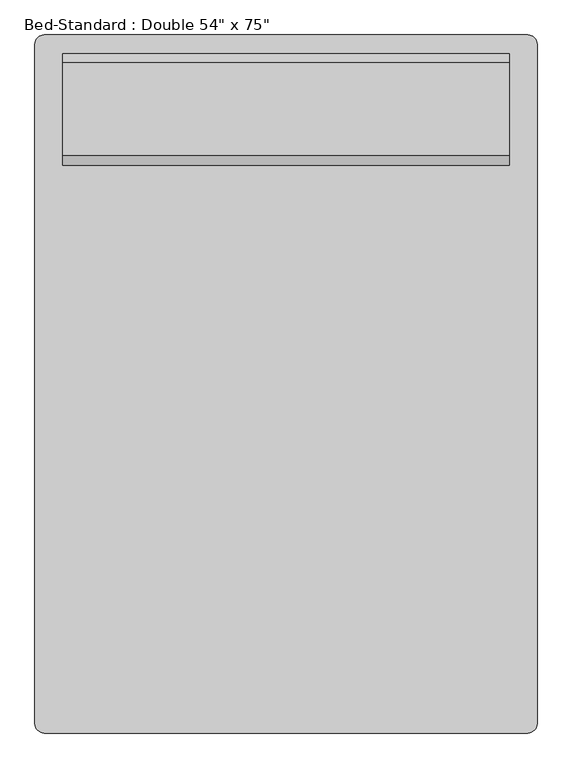
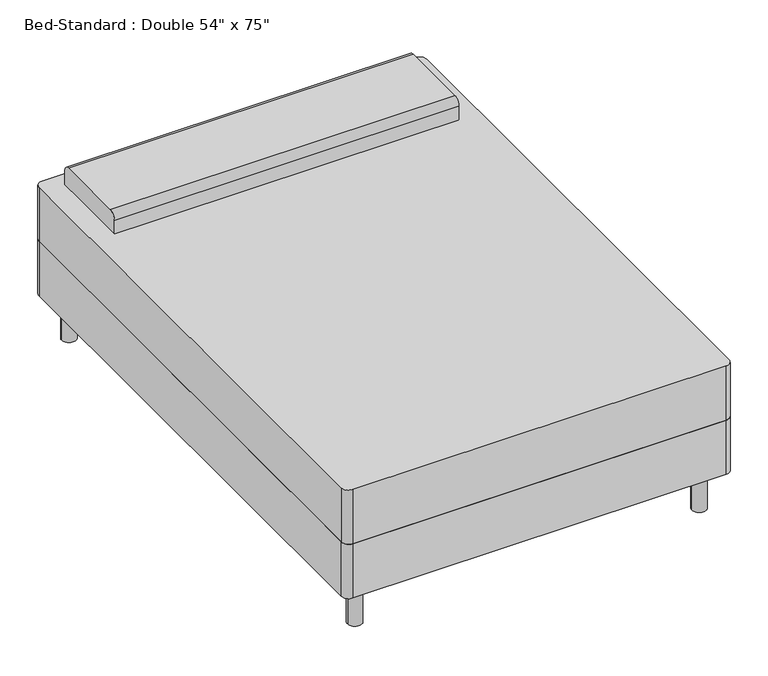
"""IFC4 building model written with IfcOpenShell, lengths in millimetres: furniture geometry."""

import ifcopenshell
import ifcopenshell.guid

model = None  # the IFC model being written
_history = None  # IfcOwnerHistory: only IFC2X3 demands one
_inside = {}  # id of a spatial element -> (the spatial element, [elements in it])
_under = {}  # id of a project, library or spatial element -> (it, [spatial elements below it])
_declared = {}  # id of a project -> (the project, [libraries it declares])
_typed = {}  # id of a type object -> (the type object, [elements of that type])
_made_of = {}  # id of a material, layer set ... -> (it, [elements and type objects made of it])


def new_model(schema):
    """Start an empty IFC model of exactly this schema.

    Asked for "IFC4X3", IfcOpenShell would pick the latest addendum, in which some entities
    have other attributes; the version numbers below select the first issue.
    IFC2X3 requires an IfcOwnerHistory on every rooted entity: one is made here for all.
    """
    global model, _history
    if schema == "IFC4X3":
        model = ifcopenshell.file(schema_version=(4, 3, 0, 0))
    else:
        model = ifcopenshell.file(schema=schema)
    _inside.clear()
    _under.clear()
    _declared.clear()
    _typed.clear()
    _made_of.clear()
    _history = None
    if model.schema == "IFC2X3":
        org = make("IfcOrganization", Name="unknown")
        user = make(
            "IfcPersonAndOrganization",
            ThePerson=make("IfcPerson", FamilyName="unknown"),
            TheOrganization=org,
        )
        app = make(
            "IfcApplication",
            ApplicationDeveloper=org,
            Version="unknown",
            ApplicationFullName="unknown",
            ApplicationIdentifier="unknown",
        )
        _history = make(
            "IfcOwnerHistory",
            OwningUser=user,
            OwningApplication=app,
            ChangeAction="ADDED",
            CreationDate=0,
        )
    return model


def make(cls, **values):
    """One entity of the class cls with the attributes given. An attribute that is None is left unset."""
    return model.create_entity(
        cls, **{name: value for name, value in values.items() if value is not None}
    )


def rooted(cls, **values):
    """An entity with a GlobalId (a new one), such as an element, a storey or a relation."""
    return make(cls, GlobalId=ifcopenshell.guid.new(), OwnerHistory=_history, **values)


def si_unit(unit_type, name, prefix=None):
    """IfcSIUnit, for example si_unit("LENGTHUNIT", "METRE", prefix="MILLI")."""
    return make("IfcSIUnit", UnitType=unit_type, Prefix=prefix, Name=name)


def assignment(units):
    """IfcUnitAssignment: the units of a project."""
    return None if units is None else make("IfcUnitAssignment", Units=units)


def point(xyz):
    """IfcCartesianPoint."""
    return None if xyz is None else make("IfcCartesianPoint", Coordinates=xyz)


def direction(xyz):
    """IfcDirection."""
    return None if xyz is None else make("IfcDirection", DirectionRatios=xyz)


def frame(location, z_axis=None, x_axis=None):
    """IfcAxis2Placement3D, a coordinate frame: its origin and axes. An axis left out is left unset."""
    return make(
        "IfcAxis2Placement3D",
        Location=point(location),
        Axis=direction(z_axis),
        RefDirection=direction(x_axis),
    )


def frame_2d(location, x_axis=None):
    """IfcAxis2Placement2D, a coordinate frame in the plane: its origin and x axis."""
    return make(
        "IfcAxis2Placement2D", Location=point(location), RefDirection=direction(x_axis)
    )


def origin():
    """The frame at (0, 0, 0) with its axes left unset."""
    return frame((0.0, 0.0, 0.0))


def origin_with_axes():
    """The frame at (0, 0, 0) with the z axis (0, 0, 1) and the x axis (1, 0, 0) written out."""
    return frame((0.0, 0.0, 0.0), z_axis=(0.0, 0.0, 1.0), x_axis=(1.0, 0.0, 0.0))


def place(relative_to, where):
    """IfcLocalPlacement: puts the frame where relative to a parent placement (None: the world)."""
    return make(
        "IfcLocalPlacement", PlacementRelTo=relative_to, RelativePlacement=where
    )


def context(
    kind, dimensions, precision=None, world=None, true_north=None, identifier=None
):
    """IfcGeometricRepresentationContext, for example the 3D "Model" context."""
    return make(
        "IfcGeometricRepresentationContext",
        ContextIdentifier=identifier,
        ContextType=kind,
        CoordinateSpaceDimension=dimensions,
        Precision=precision,
        WorldCoordinateSystem=world,
        TrueNorth=true_north,
    )


def project(units=None, contexts=None):
    """IfcProject with its units and contexts."""
    return rooted(
        "IfcProject",
        Name="project",
        RepresentationContexts=contexts,
        UnitsInContext=assignment(units),
    )


def spatial(cls, under=None, at=None, **own):
    """A site, building, storey or space (cls), placed at a placement, below another one or the project."""
    s = rooted(cls, ObjectPlacement=at, **own)
    if under is not None:
        _under.setdefault(under.id(), (under, []))[1].append(s)
    return s


def polyline(points):
    """IfcPolyline through the points."""
    return make("IfcPolyline", Points=[point(p) for p in points])


def circle_curve(where, radius):
    """IfcCircle in the frame where."""
    return make("IfcCircle", Position=where, Radius=radius)


def trimmed(basis, trim1, trim2, sense, master):
    """IfcTrimmedCurve: the piece of a basis curve between two trims."""
    return make(
        "IfcTrimmedCurve",
        BasisCurve=basis,
        Trim1=trim1,
        Trim2=trim2,
        SenseAgreement=sense,
        MasterRepresentation=master,
    )


def segment(curve, same_sense, transition):
    """IfcCompositeCurveSegment."""
    return make(
        "IfcCompositeCurveSegment",
        Transition=transition,
        SameSense=same_sense,
        ParentCurve=curve,
    )


def composite_curve(segments, self_intersect=None):
    """IfcCompositeCurve: segments joined end to end."""
    return make("IfcCompositeCurve", Segments=segments, SelfIntersect=self_intersect)


def outline(outer, holes=None, kind="AREA"):
    """IfcArbitraryClosedProfileDef: a profile drawn as a closed curve; with holes, ...WithVoids."""
    if holes is None:
        return make("IfcArbitraryClosedProfileDef", ProfileType=kind, OuterCurve=outer)
    return make(
        "IfcArbitraryProfileDefWithVoids",
        ProfileType=kind,
        OuterCurve=outer,
        InnerCurves=holes,
    )


def extrude(swept, where, along, depth):
    """IfcExtrudedAreaSolid: the profile swept, set in the frame where, extruded along a direction by depth."""
    return make(
        "IfcExtrudedAreaSolid",
        SweptArea=swept,
        Position=where,
        ExtrudedDirection=direction(along),
        Depth=depth,
    )


def shape(context_of_items, identifier, shape_type, items):
    """IfcShapeRepresentation: the items that make up one representation, for example the "Body"."""
    return make(
        "IfcShapeRepresentation",
        ContextOfItems=context_of_items,
        RepresentationIdentifier=identifier,
        RepresentationType=shape_type,
        Items=items,
    )


def source(mapping_origin, context_of_items, identifier, shape_type, items):
    """IfcRepresentationMap: a shape defined once, which mapped items show again and again."""
    return make(
        "IfcRepresentationMap",
        MappingOrigin=mapping_origin,
        MappedRepresentation=shape(context_of_items, identifier, shape_type, items),
    )


def transform(
    local_origin,
    x_axis=None,
    y_axis=None,
    z_axis=None,
    scale=None,
    scale2=None,
    scale3=None,
    uniform=True,
):
    """IfcCartesianTransformationOperator3D, or its non-uniform kind. x_axis, y_axis, z_axis: its Axis1, 2, 3."""
    if uniform:
        return make(
            "IfcCartesianTransformationOperator3D",
            Axis1=direction(x_axis),
            Axis2=direction(y_axis),
            LocalOrigin=point(local_origin),
            Scale=scale,
            Axis3=direction(z_axis),
        )
    return make(
        "IfcCartesianTransformationOperator3DnonUniform",
        Axis1=direction(x_axis),
        Axis2=direction(y_axis),
        LocalOrigin=point(local_origin),
        Scale=scale,
        Axis3=direction(z_axis),
        Scale2=scale2,
        Scale3=scale3,
    )


def mapped(mapping_source, mapping_target):
    """IfcMappedItem: shows the shape of a source again, moved by a transform."""
    return make(
        "IfcMappedItem", MappingSource=mapping_source, MappingTarget=mapping_target
    )


def made_of(thing, what):
    """Note that an element or type object is made of a material, layer set ...; save() writes the relation."""
    if what is not None:
        _made_of.setdefault(what.id(), (what, []))[1].append(thing)
    return thing


def element(
    cls,
    number,
    at=None,
    inside=None,
    cuts=None,
    type_object=None,
    material=None,
    context=None,
    identifier="Body",
    shape_type=None,
    held_by="IfcProductDefinitionShape",
    body=None,
    shapes=None,
    **own,
):
    """One element of the class cls, such as IfcWall. Its Tag is "e" and its number.

    at: its placement. inside: the storey or other place that contains it. cuts: it is an
    opening in that element (IfcRelVoidsElement). A single representation is given by context,
    identifier, shape_type and body (its items); several are given by shapes. held_by: the class
    of the entity that holds the representations. save() writes the other relations.
    """
    e = rooted(cls, Tag="e%d" % number, ObjectPlacement=at, **own)
    if body is not None:
        shapes = [shape(context, identifier, shape_type, body)]
    if shapes is not None:
        e.Representation = make(held_by, Representations=shapes)
    if inside is not None:
        _inside.setdefault(inside.id(), (inside, []))[1].append(e)
    if cuts is not None:
        rooted(
            "IfcRelVoidsElement", RelatingBuildingElement=cuts, RelatedOpeningElement=e
        )
    if type_object is not None:
        _typed.setdefault(type_object.id(), (type_object, []))[1].append(e)
    return made_of(e, material)


def aggregate(whole, parts):
    """IfcRelAggregates: a whole, such as a stair, and the parts it consists of."""
    return rooted("IfcRelAggregates", RelatingObject=whole, RelatedObjects=parts)


def save(model, path):
    """Write the relations noted so far, then the file.

    IfcRelAggregates (storeys below a building ...), IfcRelContainedInSpatialStructure (elements
    in a storey), IfcRelDefinesByType, IfcRelAssociatesMaterial and IfcRelDeclares: one each for
    every whole, place, type object, material and project.
    """
    for whole, parts in _under.values():
        aggregate(whole, parts)
    for where, things in _inside.values():
        rooted(
            "IfcRelContainedInSpatialStructure",
            RelatedElements=things,
            RelatingStructure=where,
        )
    for kind, things in _typed.values():
        rooted("IfcRelDefinesByType", RelatedObjects=things, RelatingType=kind)
    for what, things in _made_of.values():
        rooted("IfcRelAssociatesMaterial", RelatedObjects=things, RelatingMaterial=what)
    for by, libraries in _declared.values():
        rooted("IfcRelDeclares", RelatingContext=by, RelatedDefinitions=libraries)
    model.write(path)


def furniture_0253826f(model_context):
    return source(origin(), model_context, "Body", "SweptSolid", [
        extrude(outline(composite_curve([segment(polyline([(-414.3114754, -972.695082), (-414.3114754, 881.504918)]), True, "CONTINUOUS"), segment(trimmed(circle_curve(frame_2d((-388.9114754, 881.504918)), 25.4), [point((-414.3114754, 881.504918))], [point((-388.9114754, 906.904918))], False, "CARTESIAN"), True, "CONTINUOUS"), segment(polyline([(-388.9114754, 906.904918), (931.8885246, 906.904918)]), True, "CONTINUOUS"), segment(trimmed(circle_curve(frame_2d((931.8885246, 881.504918)), 25.4), [point((931.8885246, 906.904918))], [point((957.2885246, 881.504918))], False, "CARTESIAN"), True, "CONTINUOUS"), segment(polyline([(957.2885246, 881.504918), (957.2885246, -972.695082)]), True, "CONTINUOUS"), segment(trimmed(circle_curve(frame_2d((931.8885246, -972.695082)), 25.4), [point((957.2885246, -972.695082))], [point((931.8885246, -998.095082))], False, "CARTESIAN"), True, "CONTINUOUS"), segment(polyline([(931.8885246, -998.095082), (-388.9114754, -998.095082)]), True, "CONTINUOUS"), segment(trimmed(circle_curve(frame_2d((-388.9114754, -972.695082)), 25.4), [point((-388.9114754, -998.095082))], [point((-414.3114754, -972.695082))], False, "CARTESIAN"), True, "CONTINUOUS")], self_intersect=False)), frame((0.0, 0.0, 152.4), z_axis=(0.0, 0.0, 1.0), x_axis=(1.0, 0.0, 0.0)), (0.0, 0.0, 1.0), 203.2),
        extrude(outline(composite_curve([segment(polyline([(551.304918, 558.8), (551.304918, 609.6)]), True, "CONTINUOUS"), segment(trimmed(circle_curve(frame_2d((576.704918, 609.6)), 25.4), [point((551.304918, 609.6))], [point((576.704918, 635.0))], False, "CARTESIAN"), True, "CONTINUOUS"), segment(polyline([(576.704918, 635.0), (830.704918, 635.0)]), True, "CONTINUOUS"), segment(trimmed(circle_curve(frame_2d((830.704918, 609.6)), 25.4), [point((830.704918, 635.0))], [point((856.104918, 609.6))], False, "CARTESIAN"), True, "CONTINUOUS"), segment(polyline([(856.104918, 609.6), (856.104918, 558.8), (551.304918, 558.8)]), True, "CONTINUOUS")], self_intersect=False)), frame((-338.1114754, 0.0, 0.0), z_axis=(1.0, 0.0, 0.0), x_axis=(0.0, 1.0, 0.0)), (0.0, 0.0, 1.0), 1219.2),
        extrude(outline(composite_curve([segment(trimmed(circle_curve(frame_2d((-338.1114754, 830.704918)), 25.4), [point((-363.5114754, 830.704918))], [point((-312.7114754, 830.704918))], False, "CARTESIAN"), True, "CONTINUOUS"), segment(trimmed(circle_curve(frame_2d((-338.1114754, 830.704918)), 25.4), [point((-312.7114754, 830.704918))], [point((-363.5114754, 830.704918))], False, "CARTESIAN"), True, "CONTINUOUS")], self_intersect=False)), origin_with_axes(), (0.0, 0.0, 1.0), 152.4),
        extrude(outline(composite_curve([segment(trimmed(circle_curve(frame_2d((881.0885246, 830.704918)), 25.4), [point((855.6885246, 830.704918))], [point((906.4885246, 830.704918))], False, "CARTESIAN"), True, "CONTINUOUS"), segment(trimmed(circle_curve(frame_2d((881.0885246, 830.704918)), 25.4), [point((906.4885246, 830.704918))], [point((855.6885246, 830.704918))], False, "CARTESIAN"), True, "CONTINUOUS")], self_intersect=False)), origin_with_axes(), (0.0, 0.0, 1.0), 152.4),
        extrude(outline(composite_curve([segment(trimmed(circle_curve(frame_2d((881.0885246, -921.895082)), 25.4), [point((855.6885246, -921.895082))], [point((906.4885246, -921.895082))], False, "CARTESIAN"), True, "CONTINUOUS"), segment(trimmed(circle_curve(frame_2d((881.0885246, -921.895082)), 25.4), [point((906.4885246, -921.895082))], [point((855.6885246, -921.895082))], False, "CARTESIAN"), True, "CONTINUOUS")], self_intersect=False)), origin_with_axes(), (0.0, 0.0, 1.0), 152.4),
        extrude(outline(composite_curve([segment(trimmed(circle_curve(frame_2d((-338.1114754, -921.895082)), 25.4), [point((-363.5114754, -921.895082))], [point((-312.7114754, -921.895082))], False, "CARTESIAN"), True, "CONTINUOUS"), segment(trimmed(circle_curve(frame_2d((-338.1114754, -921.895082)), 25.4), [point((-312.7114754, -921.895082))], [point((-363.5114754, -921.895082))], False, "CARTESIAN"), True, "CONTINUOUS")], self_intersect=False)), origin_with_axes(), (0.0, 0.0, 1.0), 152.4),
        extrude(outline(composite_curve([segment(polyline([(-388.9114754, 906.904918), (931.8885246, 906.904918)]), True, "CONTINUOUS"), segment(trimmed(circle_curve(frame_2d((931.8885246, 881.504918)), 25.4), [point((931.8885246, 906.904918))], [point((957.2885246, 881.504918))], False, "CARTESIAN"), True, "CONTINUOUS"), segment(polyline([(957.2885246, 881.504918), (957.2885246, -972.695082)]), True, "CONTINUOUS"), segment(trimmed(circle_curve(frame_2d((931.8885246, -972.695082)), 25.4), [point((957.2885246, -972.695082))], [point((931.8885246, -998.095082))], False, "CARTESIAN"), True, "CONTINUOUS"), segment(polyline([(931.8885246, -998.095082), (-388.9114754, -998.095082)]), True, "CONTINUOUS"), segment(trimmed(circle_curve(frame_2d((-388.9114754, -972.695082)), 25.4), [point((-388.9114754, -998.095082))], [point((-414.3114754, -972.695082))], False, "CARTESIAN"), True, "CONTINUOUS"), segment(polyline([(-414.3114754, -972.695082), (-414.3114754, 881.504918)]), True, "CONTINUOUS"), segment(trimmed(circle_curve(frame_2d((-388.9114754, 881.504918)), 25.4), [point((-414.3114754, 881.504918))], [point((-388.9114754, 906.904918))], False, "CARTESIAN"), True, "CONTINUOUS")], self_intersect=False)), frame((0.0, 0.0, 355.6), z_axis=(0.0, 0.0, 1.0), x_axis=(1.0, 0.0, 0.0)), (0.0, 0.0, 1.0), 203.2),
    ])


if __name__ == "__main__":
    model = new_model("IFC4")
    model_context = context("Model", 3, world=origin())
    ifc_project = project(units=[si_unit("LENGTHUNIT", "METRE", prefix="MILLI")], contexts=[model_context])
    site = spatial("IfcSite", under=ifc_project)
    building = spatial("IfcBuilding", under=site)
    placement = place(None, origin())
    furniture_shape = furniture_0253826f(model_context)
    element("IfcFurniture", 1, ObjectType="Bed-Standard : Double 54\" x 75\"", at=placement, inside=building, context=model_context, shape_type="MappedRepresentation", body=[
        mapped(furniture_shape, transform((0.0, 0.0, 0.0), x_axis=(1.0, 0.0, 0.0), y_axis=(0.0, 1.0, 0.0), z_axis=(0.0, 0.0, 1.0))),
    ])
    save(model, "model.ifc")

# Revit data of these elements
# Project information
#   Author = "Kyle Bernhardt"
#   Project Issue Date = "Issue Date"
#   Project Status = "In Design"
#   Client Name = "Vandalay Industries"
#   Project Address = "123 Fake St\nAnytown, USA"
#   Project Name = "Urban House"
#   Project Number = "42"
#   Document GUID = "a6304091-b791-4536-90d4-6892977b827c"
#   SR Document GUID = "a504a634-f161-4fe4-96e9-0082261ef901"
# Type "Bed-Standard : Double 54\" x 75\""
#   Assembly Code = "E2020200"
#   Length = 6' - 3"
#   Width = 4' - 6"
#   Pillow Material = Textile - White
#   Frame Material = Wood - Birch
#   Leg Material = Metal - Chrome
#   Mattress Material = Textile - White
# Element 1 (IfcFurniture, "Bed-Standard : Double 54\" x 75\"")
#   Materials on its faces: "Textile - White", "Wood - Birch", "Metal - Chrome"
# Materials
#   "Textile - White": class "Unassigned", colour RGB 247 247 239, transparency 0, Comments = "Rendering appearance not upgraded Rendering appearance not upgraded "
#   "Wood - Birch": class "Wood", colour RGB 185 153 119, transparency 0, Comments = "Rendering appearance not upgraded Rendering appearance not upgraded "
#   "Metal - Chrome": class "Metal", colour RGB 244 244 244, transparency 0, Comments = "Rendering appearance not upgraded Rendering appearance not upgraded ", Description = "Chrome"
